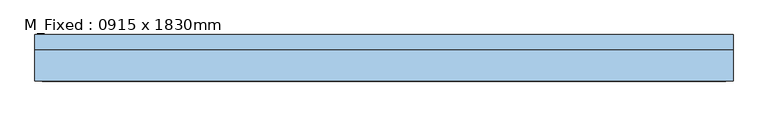
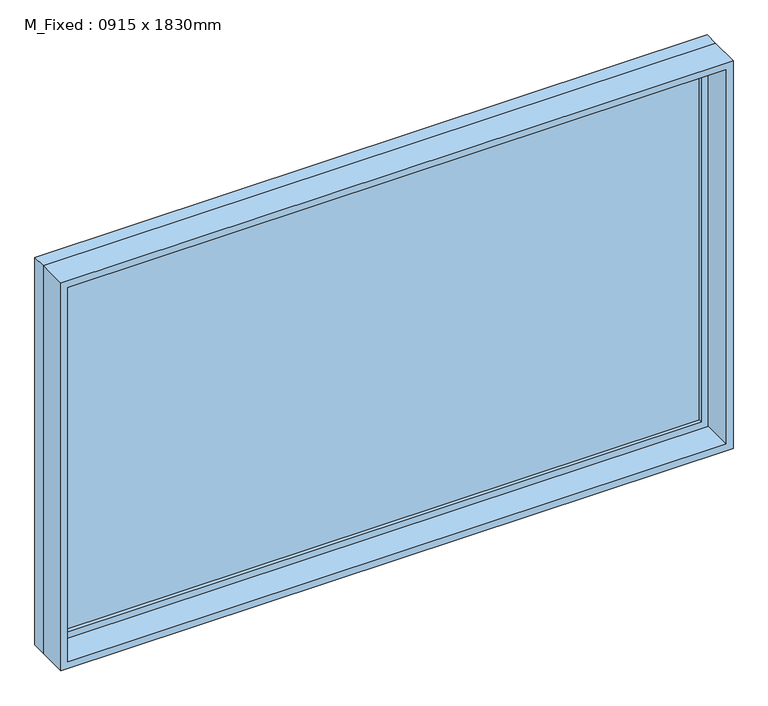
"""IFC4 building model written with IfcOpenShell, lengths in millimetres: window geometry, M_Fixed : 0915 x 1830mm."""

from ifc_helpers import new_model, si_unit, frame, origin, place, context, project, spatial, polyline, outline, extrude, source, transform, mapped, element, save


def m_fixed_0915_x_1830mm_9a0b4d00(model_context):
    return source(origin(), model_context, "Body", "SweptSolid", [
        extrude(outline(polyline([(-1437.0, 78.0), (1437.0, 78.0), (1437.0, 66.0), (-1437.0, 66.0), (-1437.0, 78.0)])), frame((0.0, 0.0, 368.0), z_axis=(0.0, 0.0, 1.0), x_axis=(1.0, 0.0, 0.0)), (0.0, 0.0, 1.0), 1704.0),
        extrude(outline(polyline([(2116.0, -1481.0), (324.0, -1481.0), (324.0, 1481.0), (2116.0, 1481.0), (2116.0, -1481.0)]), holes=[polyline([(2072.0, -1437.0), (2072.0, 1437.0), (368.0, 1437.0), (368.0, -1437.0), (2072.0, -1437.0)])]), frame((0.0, 50.0, 0.0), z_axis=(0.0, 1.0, 0.0), x_axis=(0.0, 0.0, 1.0)), (0.0, 0.0, 1.0), 44.0),
        extrude(outline(polyline([(2135.0, -1500.0), (305.0, -1500.0), (305.0, 1500.0), (2135.0, 1500.0), (2135.0, -1500.0)]), holes=[polyline([(2116.0, -1481.0), (2116.0, 1481.0), (324.0, 1481.0), (324.0, -1481.0), (2116.0, -1481.0)])]), frame((0.0, 50.0, 0.0), z_axis=(0.0, 1.0, 0.0), x_axis=(0.0, 0.0, 1.0)), (0.0, 0.0, 1.0), 63.0),
        extrude(outline(polyline([(2135.0, -1500.0), (305.0, -1500.0), (305.0, 1500.0), (2135.0, 1500.0), (2135.0, -1500.0)]), holes=[polyline([(2103.0, -1468.0), (2103.0, 1468.0), (337.0, 1468.0), (337.0, -1468.0), (2103.0, -1468.0)])]), frame((0.0, -87.0, 0.0), z_axis=(0.0, 1.0, 0.0), x_axis=(0.0, 0.0, 1.0)), (0.0, 0.0, 1.0), 137.0),
    ])


if __name__ == "__main__":
    model = new_model("IFC4")
    model_context = context("Model", 3, world=origin())
    ifc_project = project(units=[si_unit("LENGTHUNIT", "METRE", prefix="MILLI")], contexts=[model_context])
    site = spatial("IfcSite", under=ifc_project)
    building = spatial("IfcBuilding", under=site)
    placement = place(None, origin())
    m_fixed_0915_x_1830mm_shape = m_fixed_0915_x_1830mm_9a0b4d00(model_context)
    element("IfcWindow", 1, ObjectType="M_Fixed : 0915 x 1830mm", at=placement, inside=building, context=model_context, shape_type="MappedRepresentation", body=[
        mapped(m_fixed_0915_x_1830mm_shape, transform((0.0, 0.0, 0.0), x_axis=(1.0, 0.0, 0.0), y_axis=(0.0, 1.0, 0.0), z_axis=(0.0, 0.0, 1.0))),
    ])
    save(model, "model.ifc")

# Revit data of these elements
# Type "M_Fixed : 0915 x 1830mm"
#   Type Mark = "18"
#   Construction Type Id = "GSP4R"
#   Analytic Construction = "1/8 in Pilkington single glazing"
#   Visual Light Transmittance = 0.9
#   Thermal Resistance (R) = 0.271106 (m²·K)/W
#   Solar Heat Gain Coefficient = 0.78
#   Heat Transfer Coefficient (U) = 3.6886 W/(m²·K)
#   Height = 1830 mm
#   Default Sill Height = 305 mm
#   Width = 3000 mm
#   Window Inset = 19 mm
#   Frame Exterior Material = Sash
#   Frame Interior Material = Sash
#   Glass Pane Material = Glass
#   Sash = Sash
#   Wall Closure = (empty or 0)
# Element 1 (IfcWindow, "M_Fixed : 0915 x 1830mm")
#   Materials on its faces: "Sash", "Glass"
# Materials
#   "Sash": class "Wood", colour RGB 224 178 126, transparency 0, Cost = 0
#   "Glass": class "Glass", colour RGB 0 128 192, transparency 0.9, Description = "Soda Lime Glass", Cost = 0
